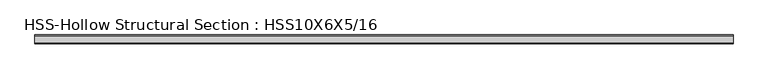
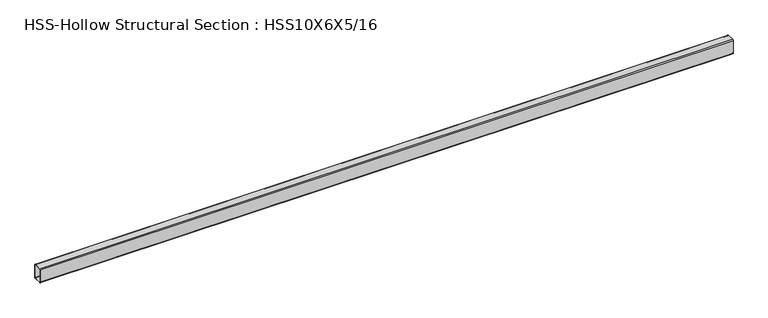
"""IFC4 building model written with IfcOpenShell, lengths in millimetres: beam geometry, HSS-Hollow Structural Section : HSS10X6X5/16."""

from ifc_helpers import new_model, si_unit, point, frame, frame_2d, origin, place, context, project, spatial, polyline, circle_curve, trimmed, segment, composite_curve, outline, extrude, source, transform, mapped, element, save


def hss_hollow_structural_section_hss10x6x5_16_48ea5751(model_context):
    return source(origin(), model_context, "Body", "SweptSolid", [
        extrude(outline(composite_curve([segment(polyline([(76.2, 112.2172), (76.2, -112.2172)]), True, "CONTINUOUS"), segment(trimmed(circle_curve(frame_2d((61.4172, -112.2172)), 14.7828), [point((76.2, -112.2172))], [point((61.4172, -127.0))], False, "CARTESIAN"), True, "CONTINUOUS"), segment(polyline([(61.4172, -127.0), (-61.4172, -127.0)]), True, "CONTINUOUS"), segment(trimmed(circle_curve(frame_2d((-61.4172, -112.2172)), 14.7828), [point((-61.4172, -127.0))], [point((-76.2, -112.2172))], False, "CARTESIAN"), True, "CONTINUOUS"), segment(polyline([(-76.2, -112.2172), (-76.2, 112.2172)]), True, "CONTINUOUS"), segment(trimmed(circle_curve(frame_2d((-61.4172, 112.2172)), 14.7828), [point((-76.2, 112.2172))], [point((-61.4172, 127.0))], False, "CARTESIAN"), True, "CONTINUOUS"), segment(polyline([(-61.4172, 127.0), (61.4172, 127.0)]), True, "CONTINUOUS"), segment(trimmed(circle_curve(frame_2d((61.4172, 112.2172)), 14.7828), [point((61.4172, 127.0))], [point((76.2, 112.2172))], False, "CARTESIAN"), True, "CONTINUOUS")], self_intersect=False), holes=[composite_curve([segment(trimmed(circle_curve(frame_2d((-61.4172, 112.2172)), 7.3914), [point((-61.4172, 119.6086))], [point((-68.8086, 112.2172))], True, "CARTESIAN"), True, "CONTINUOUS"), segment(polyline([(-68.8086, 112.2172), (-68.8086, -112.2172)]), True, "CONTINUOUS"), segment(trimmed(circle_curve(frame_2d((-61.4172, -112.2172)), 7.3914), [point((-68.8086, -112.2172))], [point((-61.4172, -119.6086))], True, "CARTESIAN"), True, "CONTINUOUS"), segment(polyline([(-61.4172, -119.6086), (61.4172, -119.6086)]), True, "CONTINUOUS"), segment(trimmed(circle_curve(frame_2d((61.4172, -112.2172)), 7.3914), [point((61.4172, -119.6086))], [point((68.8086, -112.2172))], True, "CARTESIAN"), True, "CONTINUOUS"), segment(polyline([(68.8086, -112.2172), (68.8086, 112.2172)]), True, "CONTINUOUS"), segment(trimmed(circle_curve(frame_2d((61.4172, 112.2172)), 7.3914), [point((68.8086, 112.2172))], [point((61.4172, 119.6086))], True, "CARTESIAN"), True, "CONTINUOUS"), segment(polyline([(61.4172, 119.6086), (-61.4172, 119.6086)]), True, "CONTINUOUS")], self_intersect=False)]), frame((-6018.9928962, 0.0, 0.0), z_axis=(1.0, 0.0, 0.0), x_axis=(0.0, 1.0, 0.0)), (0.0, 0.0, 1.0), 11926.8680416),
    ])


if __name__ == "__main__":
    model = new_model("IFC4")
    model_context = context("Model", 3, world=origin())
    ifc_project = project(units=[si_unit("LENGTHUNIT", "METRE", prefix="MILLI")], contexts=[model_context])
    site = spatial("IfcSite", under=ifc_project)
    building = spatial("IfcBuilding", under=site)
    placement = place(None, origin())
    hss_hollow_structural_section_hss10x6x5_16_shape = hss_hollow_structural_section_hss10x6x5_16_48ea5751(model_context)
    element("IfcBeam", 1, ObjectType="HSS-Hollow Structural Section : HSS10X6X5/16", at=placement, inside=building, context=model_context, shape_type="MappedRepresentation", body=[
        mapped(hss_hollow_structural_section_hss10x6x5_16_shape, transform((0.0, 0.0, 0.0), x_axis=(1.0, 0.0, 0.0), y_axis=(0.0, 1.0, 0.0), z_axis=(0.0, 0.0, 1.0))),
    ])
    save(model, "model.ifc")

# Revit data of these elements
# Type "HSS-Hollow Structural Section : HSS10X6X5/16"
#   Assembly Code = "B10"
#   Shape = "Rect."
#   W = 31.8
#   Ht = 0' - 10"
#   Length [instance default] = 5' - 0"
#   b = 0' - 6"
#   kr = 0' - 0.582"
#   t = 0' - 0.291"
#   A = 0.0608333 SF
#   Structural Material [instance default] = Steel ASTM A500, Grade B, Rectangular and Square
# Element 1 (IfcBeam, "HSS-Hollow Structural Section : HSS10X6X5/16")
#   Structural Material = Steel ASTM A992
#   Materials on its faces: "Steel ASTM A992"
# Materials
#   "Steel ASTM A500, Grade B, Rectangular and Square": class "Metal", colour RGB 199 199 199, transparency 0, Description = "Carbon steel", Cost = 0
#   "Steel ASTM A992": class "Metal", colour RGB 199 199 199, transparency 0, Description = "Structural steel 50ksi", Cost = 0
